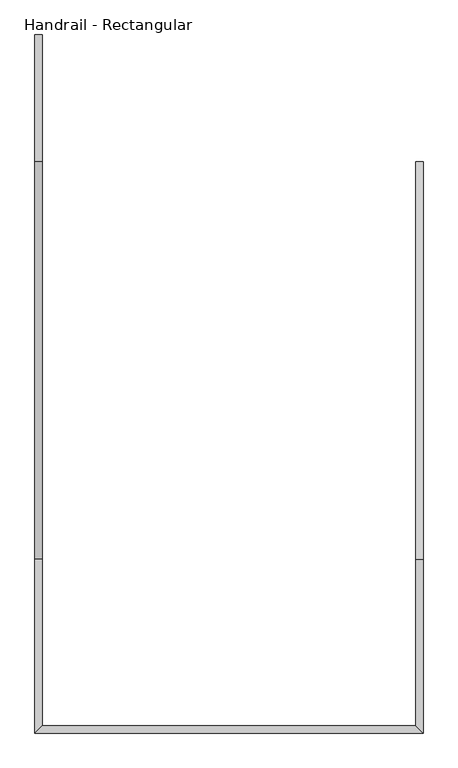
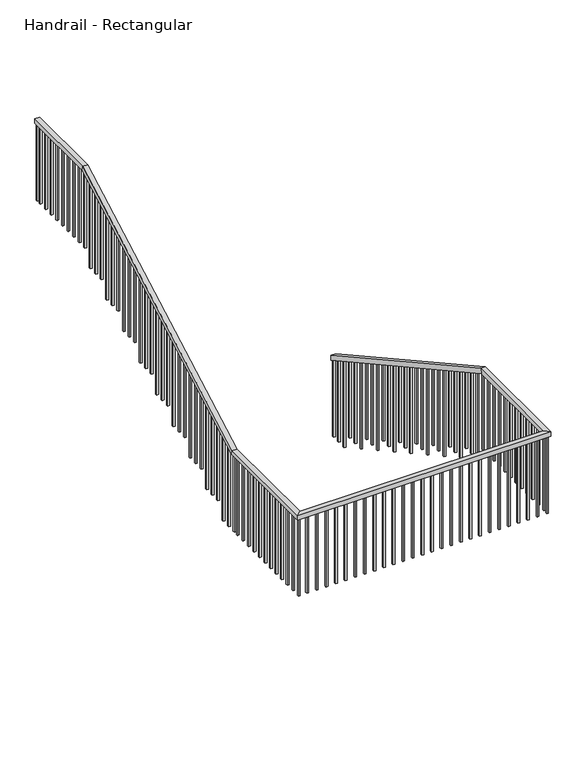
"""IFC4 building model written with IfcOpenShell, lengths in millimetres: railing geometry, Handrail - Rectangular."""

import ifcopenshell
import ifcopenshell.guid

model = None  # the IFC model being written
_history = None  # IfcOwnerHistory: only IFC2X3 demands one
_inside = {}  # id of a spatial element -> (the spatial element, [elements in it])
_under = {}  # id of a project, library or spatial element -> (it, [spatial elements below it])
_declared = {}  # id of a project -> (the project, [libraries it declares])
_typed = {}  # id of a type object -> (the type object, [elements of that type])
_made_of = {}  # id of a material, layer set ... -> (it, [elements and type objects made of it])


def new_model(schema):
    """Start an empty IFC model of exactly this schema.

    Asked for "IFC4X3", IfcOpenShell would pick the latest addendum, in which some entities
    have other attributes; the version numbers below select the first issue.
    IFC2X3 requires an IfcOwnerHistory on every rooted entity: one is made here for all.
    """
    global model, _history
    if schema == "IFC4X3":
        model = ifcopenshell.file(schema_version=(4, 3, 0, 0))
    else:
        model = ifcopenshell.file(schema=schema)
    _inside.clear()
    _under.clear()
    _declared.clear()
    _typed.clear()
    _made_of.clear()
    _history = None
    if model.schema == "IFC2X3":
        org = make("IfcOrganization", Name="unknown")
        user = make(
            "IfcPersonAndOrganization",
            ThePerson=make("IfcPerson", FamilyName="unknown"),
            TheOrganization=org,
        )
        app = make(
            "IfcApplication",
            ApplicationDeveloper=org,
            Version="unknown",
            ApplicationFullName="unknown",
            ApplicationIdentifier="unknown",
        )
        _history = make(
            "IfcOwnerHistory",
            OwningUser=user,
            OwningApplication=app,
            ChangeAction="ADDED",
            CreationDate=0,
        )
    return model


def make(cls, **values):
    """One entity of the class cls with the attributes given. An attribute that is None is left unset."""
    return model.create_entity(
        cls, **{name: value for name, value in values.items() if value is not None}
    )


def rooted(cls, **values):
    """An entity with a GlobalId (a new one), such as an element, a storey or a relation."""
    return make(cls, GlobalId=ifcopenshell.guid.new(), OwnerHistory=_history, **values)


def si_unit(unit_type, name, prefix=None):
    """IfcSIUnit, for example si_unit("LENGTHUNIT", "METRE", prefix="MILLI")."""
    return make("IfcSIUnit", UnitType=unit_type, Prefix=prefix, Name=name)


def assignment(units):
    """IfcUnitAssignment: the units of a project."""
    return None if units is None else make("IfcUnitAssignment", Units=units)


def point(xyz):
    """IfcCartesianPoint."""
    return None if xyz is None else make("IfcCartesianPoint", Coordinates=xyz)


def direction(xyz):
    """IfcDirection."""
    return None if xyz is None else make("IfcDirection", DirectionRatios=xyz)


def frame(location, z_axis=None, x_axis=None):
    """IfcAxis2Placement3D, a coordinate frame: its origin and axes. An axis left out is left unset."""
    return make(
        "IfcAxis2Placement3D",
        Location=point(location),
        Axis=direction(z_axis),
        RefDirection=direction(x_axis),
    )


def origin():
    """The frame at (0, 0, 0) with its axes left unset."""
    return frame((0.0, 0.0, 0.0))


def place(relative_to, where):
    """IfcLocalPlacement: puts the frame where relative to a parent placement (None: the world)."""
    return make(
        "IfcLocalPlacement", PlacementRelTo=relative_to, RelativePlacement=where
    )


def context(
    kind, dimensions, precision=None, world=None, true_north=None, identifier=None
):
    """IfcGeometricRepresentationContext, for example the 3D "Model" context."""
    return make(
        "IfcGeometricRepresentationContext",
        ContextIdentifier=identifier,
        ContextType=kind,
        CoordinateSpaceDimension=dimensions,
        Precision=precision,
        WorldCoordinateSystem=world,
        TrueNorth=true_north,
    )


def project(units=None, contexts=None):
    """IfcProject with its units and contexts."""
    return rooted(
        "IfcProject",
        Name="project",
        RepresentationContexts=contexts,
        UnitsInContext=assignment(units),
    )


def spatial(cls, under=None, at=None, **own):
    """A site, building, storey or space (cls), placed at a placement, below another one or the project."""
    s = rooted(cls, ObjectPlacement=at, **own)
    if under is not None:
        _under.setdefault(under.id(), (under, []))[1].append(s)
    return s


def polyline(points):
    """IfcPolyline through the points."""
    return make("IfcPolyline", Points=[point(p) for p in points])


def outline(outer, holes=None, kind="AREA"):
    """IfcArbitraryClosedProfileDef: a profile drawn as a closed curve; with holes, ...WithVoids."""
    if holes is None:
        return make("IfcArbitraryClosedProfileDef", ProfileType=kind, OuterCurve=outer)
    return make(
        "IfcArbitraryProfileDefWithVoids",
        ProfileType=kind,
        OuterCurve=outer,
        InnerCurves=holes,
    )


def extrude(swept, where, along, depth):
    """IfcExtrudedAreaSolid: the profile swept, set in the frame where, extruded along a direction by depth."""
    return make(
        "IfcExtrudedAreaSolid",
        SweptArea=swept,
        Position=where,
        ExtrudedDirection=direction(along),
        Depth=depth,
    )


def faces_of(points, faces, orient=None, outer=None):
    """IfcFace entities. A face is a list of loops; a loop is a list of indices into points, from 0.

    orient and outer hold one flag for each loop. By default every Orientation is true, the
    first loop of a face is its IfcFaceOuterBound and the others are IfcFaceBound.
    """
    made = []
    for i, loops in enumerate(faces):
        bounds = []
        for j, loop in enumerate(loops):
            is_outer = j == 0 if outer is None else outer[i][j]
            bounds.append(
                make(
                    "IfcFaceOuterBound" if is_outer else "IfcFaceBound",
                    Bound=make("IfcPolyLoop", Polygon=[points[k] for k in loop]),
                    Orientation=True if orient is None else orient[i][j],
                )
            )
        made.append(make("IfcFace", Bounds=bounds))
    return made


def faceted_brep(points, faces, orient=None, outer=None, voids=None):
    """IfcFacetedBrep: a solid bounded by flat faces; with voids (closed shells), ...WithVoids."""
    shared = [point(p) for p in points]
    hull = make("IfcClosedShell", CfsFaces=faces_of(shared, faces, orient, outer))
    if voids is None:
        return make("IfcFacetedBrep", Outer=hull)
    return make(
        "IfcFacetedBrepWithVoids",
        Outer=hull,
        Voids=[
            make(cls, CfsFaces=faces_of(shared, fs, o, b)) for cls, fs, o, b in voids
        ],
    )


def shape(context_of_items, identifier, shape_type, items):
    """IfcShapeRepresentation: the items that make up one representation, for example the "Body"."""
    return make(
        "IfcShapeRepresentation",
        ContextOfItems=context_of_items,
        RepresentationIdentifier=identifier,
        RepresentationType=shape_type,
        Items=items,
    )


def source(mapping_origin, context_of_items, identifier, shape_type, items):
    """IfcRepresentationMap: a shape defined once, which mapped items show again and again."""
    return make(
        "IfcRepresentationMap",
        MappingOrigin=mapping_origin,
        MappedRepresentation=shape(context_of_items, identifier, shape_type, items),
    )


def transform(
    local_origin,
    x_axis=None,
    y_axis=None,
    z_axis=None,
    scale=None,
    scale2=None,
    scale3=None,
    uniform=True,
):
    """IfcCartesianTransformationOperator3D, or its non-uniform kind. x_axis, y_axis, z_axis: its Axis1, 2, 3."""
    if uniform:
        return make(
            "IfcCartesianTransformationOperator3D",
            Axis1=direction(x_axis),
            Axis2=direction(y_axis),
            LocalOrigin=point(local_origin),
            Scale=scale,
            Axis3=direction(z_axis),
        )
    return make(
        "IfcCartesianTransformationOperator3DnonUniform",
        Axis1=direction(x_axis),
        Axis2=direction(y_axis),
        LocalOrigin=point(local_origin),
        Scale=scale,
        Axis3=direction(z_axis),
        Scale2=scale2,
        Scale3=scale3,
    )


def mapped(mapping_source, mapping_target):
    """IfcMappedItem: shows the shape of a source again, moved by a transform."""
    return make(
        "IfcMappedItem", MappingSource=mapping_source, MappingTarget=mapping_target
    )


def made_of(thing, what):
    """Note that an element or type object is made of a material, layer set ...; save() writes the relation."""
    if what is not None:
        _made_of.setdefault(what.id(), (what, []))[1].append(thing)
    return thing


def element(
    cls,
    number,
    at=None,
    inside=None,
    cuts=None,
    type_object=None,
    material=None,
    context=None,
    identifier="Body",
    shape_type=None,
    held_by="IfcProductDefinitionShape",
    body=None,
    shapes=None,
    **own,
):
    """One element of the class cls, such as IfcWall. Its Tag is "e" and its number.

    at: its placement. inside: the storey or other place that contains it. cuts: it is an
    opening in that element (IfcRelVoidsElement). A single representation is given by context,
    identifier, shape_type and body (its items); several are given by shapes. held_by: the class
    of the entity that holds the representations. save() writes the other relations.
    """
    e = rooted(cls, Tag="e%d" % number, ObjectPlacement=at, **own)
    if body is not None:
        shapes = [shape(context, identifier, shape_type, body)]
    if shapes is not None:
        e.Representation = make(held_by, Representations=shapes)
    if inside is not None:
        _inside.setdefault(inside.id(), (inside, []))[1].append(e)
    if cuts is not None:
        rooted(
            "IfcRelVoidsElement", RelatingBuildingElement=cuts, RelatedOpeningElement=e
        )
    if type_object is not None:
        _typed.setdefault(type_object.id(), (type_object, []))[1].append(e)
    return made_of(e, material)


def aggregate(whole, parts):
    """IfcRelAggregates: a whole, such as a stair, and the parts it consists of."""
    return rooted("IfcRelAggregates", RelatingObject=whole, RelatedObjects=parts)


def save(model, path):
    """Write the relations noted so far, then the file.

    IfcRelAggregates (storeys below a building ...), IfcRelContainedInSpatialStructure (elements
    in a storey), IfcRelDefinesByType, IfcRelAssociatesMaterial and IfcRelDeclares: one each for
    every whole, place, type object, material and project.
    """
    for whole, parts in _under.values():
        aggregate(whole, parts)
    for where, things in _inside.values():
        rooted(
            "IfcRelContainedInSpatialStructure",
            RelatedElements=things,
            RelatingStructure=where,
        )
    for kind, things in _typed.values():
        rooted("IfcRelDefinesByType", RelatedObjects=things, RelatingType=kind)
    for what, things in _made_of.values():
        rooted("IfcRelAssociatesMaterial", RelatedObjects=things, RelatingMaterial=what)
    for by, libraries in _declared.values():
        rooted("IfcRelDeclares", RelatingContext=by, RelatedDefinitions=libraries)
    model.write(path)


def handrail_rectangular_0e0fe6d2(model_context):
    return source(origin(), model_context, "Body", "SolidModel", [
        faceted_brep([(-73320.227375, 12915.9, 10449.0921053), (-73269.427375, 12915.9, 10449.0921053), (-73269.427375, 12915.9, 10391.0509841), (-73320.227375, 12915.9, 10391.0509841), (-73320.227375, 10172.7, 11965.0710526), (-73269.427375, 10172.7, 11965.0710526), (-73269.427375, 10159.5970189, 11914.2710526), (-73320.227375, 10159.5970189, 11914.2710526), (-73320.227375, 9023.35, 11965.0710526), (-73269.427375, 8972.55, 11965.0710526), (-73269.427375, 8972.55, 11914.2710526), (-73320.227375, 9023.35, 11914.2710526), (-75898.327375, 9023.35, 11965.0710526), (-75949.127375, 8972.55, 11965.0710526), (-75949.127375, 8972.55, 11914.2710526), (-75898.327375, 9023.35, 11914.2710526), (-75898.327375, 10172.7, 11965.0710526), (-75949.127375, 10172.7, 11965.0710526), (-75949.127375, 10185.8029811, 11914.2710526), (-75898.327375, 10185.8029811, 11914.2710526), (-75898.327375, 12915.9, 13481.05), (-75949.127375, 12915.9, 13481.05), (-75949.127375, 12929.0029811, 13430.25), (-75898.327375, 12929.0029811, 13430.25), (-75898.327375, 13792.2, 13481.05), (-75898.327375, 13792.2, 13430.25), (-75949.127375, 13792.2, 13430.25), (-75949.127375, 13792.2, 13481.05)], [[[0, 1, 2, 3]], [[1, 0, 4, 5]], [[2, 1, 5, 6]], [[3, 2, 6, 7]], [[0, 3, 7, 4]], [[5, 4, 8, 9]], [[6, 5, 9, 10]], [[7, 6, 10, 11]], [[4, 7, 11, 8]], [[9, 8, 12, 13]], [[10, 9, 13, 14]], [[11, 10, 14, 15]], [[8, 11, 15, 12]], [[13, 12, 16, 17]], [[14, 13, 17, 18]], [[15, 14, 18, 19]], [[12, 15, 19, 16]], [[17, 16, 20, 21]], [[18, 17, 21, 22]], [[19, 18, 22, 23]], [[16, 19, 23, 20]], [[24, 25, 26, 27]], [[21, 20, 24, 27]], [[22, 21, 27, 26]], [[23, 22, 26, 25]], [[20, 23, 25, 24]]]),
        extrude(outline(polyline([(-75914.202375, 13719.175), (-75933.252375, 13719.175), (-75933.252375, 13738.225), (-75914.202375, 13738.225), (-75914.202375, 13719.175)])), frame((0.0, 0.0, 12566.65), z_axis=(0.0, 0.0, 1.0), x_axis=(1.0, 0.0, 0.0)), (0.0, 0.0, 1.0), 863.6),
        extrude(outline(polyline([(-75914.202375, 13617.575), (-75933.252375, 13617.575), (-75933.252375, 13636.625), (-75914.202375, 13636.625), (-75914.202375, 13617.575)])), frame((0.0, 0.0, 12566.65), z_axis=(0.0, 0.0, 1.0), x_axis=(1.0, 0.0, 0.0)), (0.0, 0.0, 1.0), 863.6),
        extrude(outline(polyline([(-75914.202375, 13515.975), (-75933.252375, 13515.975), (-75933.252375, 13535.025), (-75914.202375, 13535.025), (-75914.202375, 13515.975)])), frame((0.0, 0.0, 12566.65), z_axis=(0.0, 0.0, 1.0), x_axis=(1.0, 0.0, 0.0)), (0.0, 0.0, 1.0), 863.6),
        extrude(outline(polyline([(-75914.202375, 13414.375), (-75933.252375, 13414.375), (-75933.252375, 13433.425), (-75914.202375, 13433.425), (-75914.202375, 13414.375)])), frame((0.0, 0.0, 12566.65), z_axis=(0.0, 0.0, 1.0), x_axis=(1.0, 0.0, 0.0)), (0.0, 0.0, 1.0), 863.6),
        extrude(outline(polyline([(-75914.202375, 13312.775), (-75933.252375, 13312.775), (-75933.252375, 13331.825), (-75914.202375, 13331.825), (-75914.202375, 13312.775)])), frame((0.0, 0.0, 12566.65), z_axis=(0.0, 0.0, 1.0), x_axis=(1.0, 0.0, 0.0)), (0.0, 0.0, 1.0), 863.6),
        extrude(outline(polyline([(-75914.202375, 13211.175), (-75933.252375, 13211.175), (-75933.252375, 13230.225), (-75914.202375, 13230.225), (-75914.202375, 13211.175)])), frame((0.0, 0.0, 12566.65), z_axis=(0.0, 0.0, 1.0), x_axis=(1.0, 0.0, 0.0)), (0.0, 0.0, 1.0), 863.6),
        extrude(outline(polyline([(-75914.202375, 13109.575), (-75933.252375, 13109.575), (-75933.252375, 13128.625), (-75914.202375, 13128.625), (-75914.202375, 13109.575)])), frame((0.0, 0.0, 12566.65), z_axis=(0.0, 0.0, 1.0), x_axis=(1.0, 0.0, 0.0)), (0.0, 0.0, 1.0), 863.6),
        extrude(outline(polyline([(-75914.202375, 13007.975), (-75933.252375, 13007.975), (-75933.252375, 13027.025), (-75914.202375, 13027.025), (-75914.202375, 13007.975)])), frame((0.0, 0.0, 12566.65), z_axis=(0.0, 0.0, 1.0), x_axis=(1.0, 0.0, 0.0)), (0.0, 0.0, 1.0), 863.6),
        extrude(outline(polyline([(12804.775, 13361.5976946), (12823.825, 13372.1253262), (12823.825, 12398.2078947), (12804.775, 12398.2078947), (12804.775, 13361.5976946)])), frame((-75933.252375, 0.0, 0.0), z_axis=(1.0, 0.0, 0.0), x_axis=(0.0, 1.0, 0.0)), (0.0, 0.0, 1.0), 19.05),
        extrude(outline(polyline([(12703.175, 13305.4503262), (12722.225, 13315.9779578), (12722.225, 12398.2078947), (12703.175, 12398.2078947), (12703.175, 13305.4503262)])), frame((-75933.252375, 0.0, 0.0), z_axis=(1.0, 0.0, 0.0), x_axis=(0.0, 1.0, 0.0)), (0.0, 0.0, 1.0), 19.05),
        extrude(outline(polyline([(12601.575, 13249.3029578), (12620.625, 13259.8305894), (12620.625, 12398.2078947), (12601.575, 12398.2078947), (12601.575, 13249.3029578)])), frame((-75933.252375, 0.0, 0.0), z_axis=(1.0, 0.0, 0.0), x_axis=(0.0, 1.0, 0.0)), (0.0, 0.0, 1.0), 19.05),
        extrude(outline(polyline([(12499.975, 13193.1555894), (12519.025, 13203.6832209), (12519.025, 12229.7657895), (12499.975, 12229.7657895), (12499.975, 13193.1555894)])), frame((-75933.252375, 0.0, 0.0), z_axis=(1.0, 0.0, 0.0), x_axis=(0.0, 1.0, 0.0)), (0.0, 0.0, 1.0), 19.05),
        extrude(outline(polyline([(12398.375, 13137.0082209), (12417.425, 13147.5358525), (12417.425, 12229.7657895), (12398.375, 12229.7657895), (12398.375, 13137.0082209)])), frame((-75933.252375, 0.0, 0.0), z_axis=(1.0, 0.0, 0.0), x_axis=(0.0, 1.0, 0.0)), (0.0, 0.0, 1.0), 19.05),
        extrude(outline(polyline([(12296.775, 13080.8608525), (12315.825, 13091.3884841), (12315.825, 12229.7657895), (12296.775, 12229.7657895), (12296.775, 13080.8608525)])), frame((-75933.252375, 0.0, 0.0), z_axis=(1.0, 0.0, 0.0), x_axis=(0.0, 1.0, 0.0)), (0.0, 0.0, 1.0), 19.05),
        extrude(outline(polyline([(12195.175, 13024.7134841), (12214.225, 13035.2411157), (12214.225, 12061.3236842), (12195.175, 12061.3236842), (12195.175, 13024.7134841)])), frame((-75933.252375, 0.0, 0.0), z_axis=(1.0, 0.0, 0.0), x_axis=(0.0, 1.0, 0.0)), (0.0, 0.0, 1.0), 19.05),
        extrude(outline(polyline([(12093.575, 12968.5661157), (12112.625, 12979.0937473), (12112.625, 12061.3236842), (12093.575, 12061.3236842), (12093.575, 12968.5661157)])), frame((-75933.252375, 0.0, 0.0), z_axis=(1.0, 0.0, 0.0), x_axis=(0.0, 1.0, 0.0)), (0.0, 0.0, 1.0), 19.05),
        extrude(outline(polyline([(11991.975, 12912.4187473), (12011.025, 12922.9463788), (12011.025, 12061.3236842), (11991.975, 12061.3236842), (11991.975, 12912.4187473)])), frame((-75933.252375, 0.0, 0.0), z_axis=(1.0, 0.0, 0.0), x_axis=(0.0, 1.0, 0.0)), (0.0, 0.0, 1.0), 19.05),
        extrude(outline(polyline([(11890.375, 12856.2713788), (11909.425, 12866.7990104), (11909.425, 11892.8815789), (11890.375, 11892.8815789), (11890.375, 12856.2713788)])), frame((-75933.252375, 0.0, 0.0), z_axis=(1.0, 0.0, 0.0), x_axis=(0.0, 1.0, 0.0)), (0.0, 0.0, 1.0), 19.05),
        extrude(outline(polyline([(11788.775, 12800.1240104), (11807.825, 12810.651642), (11807.825, 11892.8815789), (11788.775, 11892.8815789), (11788.775, 12800.1240104)])), frame((-75933.252375, 0.0, 0.0), z_axis=(1.0, 0.0, 0.0), x_axis=(0.0, 1.0, 0.0)), (0.0, 0.0, 1.0), 19.05),
        extrude(outline(polyline([(11687.175, 12743.976642), (11706.225, 12754.5042736), (11706.225, 11892.8815789), (11687.175, 11892.8815789), (11687.175, 12743.976642)])), frame((-75933.252375, 0.0, 0.0), z_axis=(1.0, 0.0, 0.0), x_axis=(0.0, 1.0, 0.0)), (0.0, 0.0, 1.0), 19.05),
        extrude(outline(polyline([(11585.575, 12687.8292736), (11604.625, 12698.3569052), (11604.625, 11724.4394737), (11585.575, 11724.4394737), (11585.575, 12687.8292736)])), frame((-75933.252375, 0.0, 0.0), z_axis=(1.0, 0.0, 0.0), x_axis=(0.0, 1.0, 0.0)), (0.0, 0.0, 1.0), 19.05),
        extrude(outline(polyline([(11483.975, 12631.6819052), (11503.025, 12642.2095367), (11503.025, 11724.4394737), (11483.975, 11724.4394737), (11483.975, 12631.6819052)])), frame((-75933.252375, 0.0, 0.0), z_axis=(1.0, 0.0, 0.0), x_axis=(0.0, 1.0, 0.0)), (0.0, 0.0, 1.0), 19.05),
        extrude(outline(polyline([(11382.375, 12575.5345367), (11401.425, 12586.0621683), (11401.425, 11724.4394737), (11382.375, 11724.4394737), (11382.375, 12575.5345367)])), frame((-75933.252375, 0.0, 0.0), z_axis=(1.0, 0.0, 0.0), x_axis=(0.0, 1.0, 0.0)), (0.0, 0.0, 1.0), 19.05),
        extrude(outline(polyline([(11280.775, 12519.3871683), (11299.825, 12529.9147999), (11299.825, 11555.9973684), (11280.775, 11555.9973684), (11280.775, 12519.3871683)])), frame((-75933.252375, 0.0, 0.0), z_axis=(1.0, 0.0, 0.0), x_axis=(0.0, 1.0, 0.0)), (0.0, 0.0, 1.0), 19.05),
        extrude(outline(polyline([(11179.175, 12463.2397999), (11198.225, 12473.7674315), (11198.225, 11555.9973684), (11179.175, 11555.9973684), (11179.175, 12463.2397999)])), frame((-75933.252375, 0.0, 0.0), z_axis=(1.0, 0.0, 0.0), x_axis=(0.0, 1.0, 0.0)), (0.0, 0.0, 1.0), 19.05),
        extrude(outline(polyline([(11077.575, 12407.0924315), (11096.625, 12417.6200631), (11096.625, 11555.9973684), (11077.575, 11555.9973684), (11077.575, 12407.0924315)])), frame((-75933.252375, 0.0, 0.0), z_axis=(1.0, 0.0, 0.0), x_axis=(0.0, 1.0, 0.0)), (0.0, 0.0, 1.0), 19.05),
        extrude(outline(polyline([(10975.975, 12350.9450631), (10995.025, 12361.4726946), (10995.025, 11387.5552632), (10975.975, 11387.5552632), (10975.975, 12350.9450631)])), frame((-75933.252375, 0.0, 0.0), z_axis=(1.0, 0.0, 0.0), x_axis=(0.0, 1.0, 0.0)), (0.0, 0.0, 1.0), 19.05),
        extrude(outline(polyline([(10874.375, 12294.7976946), (10893.425, 12305.3253262), (10893.425, 11387.5552632), (10874.375, 11387.5552632), (10874.375, 12294.7976946)])), frame((-75933.252375, 0.0, 0.0), z_axis=(1.0, 0.0, 0.0), x_axis=(0.0, 1.0, 0.0)), (0.0, 0.0, 1.0), 19.05),
        extrude(outline(polyline([(10772.775, 12238.6503262), (10791.825, 12249.1779578), (10791.825, 11387.5552632), (10772.775, 11387.5552632), (10772.775, 12238.6503262)])), frame((-75933.252375, 0.0, 0.0), z_axis=(1.0, 0.0, 0.0), x_axis=(0.0, 1.0, 0.0)), (0.0, 0.0, 1.0), 19.05),
        extrude(outline(polyline([(10671.175, 12182.5029578), (10690.225, 12193.0305894), (10690.225, 11219.1131579), (10671.175, 11219.1131579), (10671.175, 12182.5029578)])), frame((-75933.252375, 0.0, 0.0), z_axis=(1.0, 0.0, 0.0), x_axis=(0.0, 1.0, 0.0)), (0.0, 0.0, 1.0), 19.05),
        extrude(outline(polyline([(10569.575, 12126.3555894), (10588.625, 12136.8832209), (10588.625, 11219.1131579), (10569.575, 11219.1131579), (10569.575, 12126.3555894)])), frame((-75933.252375, 0.0, 0.0), z_axis=(1.0, 0.0, 0.0), x_axis=(0.0, 1.0, 0.0)), (0.0, 0.0, 1.0), 19.05),
        extrude(outline(polyline([(10467.975, 12070.2082209), (10487.025, 12080.7358525), (10487.025, 11219.1131579), (10467.975, 11219.1131579), (10467.975, 12070.2082209)])), frame((-75933.252375, 0.0, 0.0), z_axis=(1.0, 0.0, 0.0), x_axis=(0.0, 1.0, 0.0)), (0.0, 0.0, 1.0), 19.05),
        extrude(outline(polyline([(10366.375, 12014.0608525), (10385.425, 12024.5884841), (10385.425, 11050.6710526), (10366.375, 11050.6710526), (10366.375, 12014.0608525)])), frame((-75933.252375, 0.0, 0.0), z_axis=(1.0, 0.0, 0.0), x_axis=(0.0, 1.0, 0.0)), (0.0, 0.0, 1.0), 19.05),
        extrude(outline(polyline([(10264.775, 11957.9134841), (10283.825, 11968.4411157), (10283.825, 11050.6710526), (10264.775, 11050.6710526), (10264.775, 11957.9134841)])), frame((-75933.252375, 0.0, 0.0), z_axis=(1.0, 0.0, 0.0), x_axis=(0.0, 1.0, 0.0)), (0.0, 0.0, 1.0), 19.05),
        extrude(outline(polyline([(-75914.202375, 10106.025), (-75933.252375, 10106.025), (-75933.252375, 10125.075), (-75914.202375, 10125.075), (-75914.202375, 10106.025)])), frame((0.0, 0.0, 11050.6710526), z_axis=(0.0, 0.0, 1.0), x_axis=(1.0, 0.0, 0.0)), (0.0, 0.0, 1.0), 863.6),
        extrude(outline(polyline([(-75914.202375, 10004.425), (-75933.252375, 10004.425), (-75933.252375, 10023.475), (-75914.202375, 10023.475), (-75914.202375, 10004.425)])), frame((0.0, 0.0, 11050.6710526), z_axis=(0.0, 0.0, 1.0), x_axis=(1.0, 0.0, 0.0)), (0.0, 0.0, 1.0), 863.6),
        extrude(outline(polyline([(-75914.202375, 9902.825), (-75933.252375, 9902.825), (-75933.252375, 9921.875), (-75914.202375, 9921.875), (-75914.202375, 9902.825)])), frame((0.0, 0.0, 11050.6710526), z_axis=(0.0, 0.0, 1.0), x_axis=(1.0, 0.0, 0.0)), (0.0, 0.0, 1.0), 863.6),
        extrude(outline(polyline([(-75914.202375, 9801.225), (-75933.252375, 9801.225), (-75933.252375, 9820.275), (-75914.202375, 9820.275), (-75914.202375, 9801.225)])), frame((0.0, 0.0, 11050.6710526), z_axis=(0.0, 0.0, 1.0), x_axis=(1.0, 0.0, 0.0)), (0.0, 0.0, 1.0), 863.6),
        extrude(outline(polyline([(-75914.202375, 9699.625), (-75933.252375, 9699.625), (-75933.252375, 9718.675), (-75914.202375, 9718.675), (-75914.202375, 9699.625)])), frame((0.0, 0.0, 11050.6710526), z_axis=(0.0, 0.0, 1.0), x_axis=(1.0, 0.0, 0.0)), (0.0, 0.0, 1.0), 863.6),
        extrude(outline(polyline([(-75914.202375, 9598.025), (-75933.252375, 9598.025), (-75933.252375, 9617.075), (-75914.202375, 9617.075), (-75914.202375, 9598.025)])), frame((0.0, 0.0, 11050.6710526), z_axis=(0.0, 0.0, 1.0), x_axis=(1.0, 0.0, 0.0)), (0.0, 0.0, 1.0), 863.6),
        extrude(outline(polyline([(-75914.202375, 9496.425), (-75933.252375, 9496.425), (-75933.252375, 9515.475), (-75914.202375, 9515.475), (-75914.202375, 9496.425)])), frame((0.0, 0.0, 11050.6710526), z_axis=(0.0, 0.0, 1.0), x_axis=(1.0, 0.0, 0.0)), (0.0, 0.0, 1.0), 863.6),
        extrude(outline(polyline([(-75914.202375, 9394.825), (-75933.252375, 9394.825), (-75933.252375, 9413.875), (-75914.202375, 9413.875), (-75914.202375, 9394.825)])), frame((0.0, 0.0, 11050.6710526), z_axis=(0.0, 0.0, 1.0), x_axis=(1.0, 0.0, 0.0)), (0.0, 0.0, 1.0), 863.6),
        extrude(outline(polyline([(-75914.202375, 9293.225), (-75933.252375, 9293.225), (-75933.252375, 9312.275), (-75914.202375, 9312.275), (-75914.202375, 9293.225)])), frame((0.0, 0.0, 11050.6710526), z_axis=(0.0, 0.0, 1.0), x_axis=(1.0, 0.0, 0.0)), (0.0, 0.0, 1.0), 863.6),
        extrude(outline(polyline([(-75914.202375, 9191.625), (-75933.252375, 9191.625), (-75933.252375, 9210.675), (-75914.202375, 9210.675), (-75914.202375, 9191.625)])), frame((0.0, 0.0, 11050.6710526), z_axis=(0.0, 0.0, 1.0), x_axis=(1.0, 0.0, 0.0)), (0.0, 0.0, 1.0), 863.6),
        extrude(outline(polyline([(-75914.202375, 9090.025), (-75933.252375, 9090.025), (-75933.252375, 9109.075), (-75914.202375, 9109.075), (-75914.202375, 9090.025)])), frame((0.0, 0.0, 11050.6710526), z_axis=(0.0, 0.0, 1.0), x_axis=(1.0, 0.0, 0.0)), (0.0, 0.0, 1.0), 863.6),
        extrude(outline(polyline([(-75825.302375, 9007.475), (-75825.302375, 8988.425), (-75844.352375, 8988.425), (-75844.352375, 9007.475), (-75825.302375, 9007.475)])), frame((0.0, 0.0, 11050.6710526), z_axis=(0.0, 0.0, 1.0), x_axis=(1.0, 0.0, 0.0)), (0.0, 0.0, 1.0), 863.6),
        extrude(outline(polyline([(-75723.702375, 9007.475), (-75723.702375, 8988.425), (-75742.752375, 8988.425), (-75742.752375, 9007.475), (-75723.702375, 9007.475)])), frame((0.0, 0.0, 11050.6710526), z_axis=(0.0, 0.0, 1.0), x_axis=(1.0, 0.0, 0.0)), (0.0, 0.0, 1.0), 863.6),
        extrude(outline(polyline([(-75622.102375, 9007.475), (-75622.102375, 8988.425), (-75641.152375, 8988.425), (-75641.152375, 9007.475), (-75622.102375, 9007.475)])), frame((0.0, 0.0, 11050.6710526), z_axis=(0.0, 0.0, 1.0), x_axis=(1.0, 0.0, 0.0)), (0.0, 0.0, 1.0), 863.6),
        extrude(outline(polyline([(-75520.502375, 9007.475), (-75520.502375, 8988.425), (-75539.552375, 8988.425), (-75539.552375, 9007.475), (-75520.502375, 9007.475)])), frame((0.0, 0.0, 11050.6710526), z_axis=(0.0, 0.0, 1.0), x_axis=(1.0, 0.0, 0.0)), (0.0, 0.0, 1.0), 863.6),
        extrude(outline(polyline([(-75418.902375, 9007.475), (-75418.902375, 8988.425), (-75437.952375, 8988.425), (-75437.952375, 9007.475), (-75418.902375, 9007.475)])), frame((0.0, 0.0, 11050.6710526), z_axis=(0.0, 0.0, 1.0), x_axis=(1.0, 0.0, 0.0)), (0.0, 0.0, 1.0), 863.6),
        extrude(outline(polyline([(-75317.302375, 9007.475), (-75317.302375, 8988.425), (-75336.352375, 8988.425), (-75336.352375, 9007.475), (-75317.302375, 9007.475)])), frame((0.0, 0.0, 11050.6710526), z_axis=(0.0, 0.0, 1.0), x_axis=(1.0, 0.0, 0.0)), (0.0, 0.0, 1.0), 863.6),
        extrude(outline(polyline([(-75215.702375, 9007.475), (-75215.702375, 8988.425), (-75234.752375, 8988.425), (-75234.752375, 9007.475), (-75215.702375, 9007.475)])), frame((0.0, 0.0, 11050.6710526), z_axis=(0.0, 0.0, 1.0), x_axis=(1.0, 0.0, 0.0)), (0.0, 0.0, 1.0), 863.6),
        extrude(outline(polyline([(-75114.102375, 9007.475), (-75114.102375, 8988.425), (-75133.152375, 8988.425), (-75133.152375, 9007.475), (-75114.102375, 9007.475)])), frame((0.0, 0.0, 11050.6710526), z_axis=(0.0, 0.0, 1.0), x_axis=(1.0, 0.0, 0.0)), (0.0, 0.0, 1.0), 863.6),
        extrude(outline(polyline([(-75012.502375, 9007.475), (-75012.502375, 8988.425), (-75031.552375, 8988.425), (-75031.552375, 9007.475), (-75012.502375, 9007.475)])), frame((0.0, 0.0, 11050.6710526), z_axis=(0.0, 0.0, 1.0), x_axis=(1.0, 0.0, 0.0)), (0.0, 0.0, 1.0), 863.6),
        extrude(outline(polyline([(-74910.902375, 9007.475), (-74910.902375, 8988.425), (-74929.952375, 8988.425), (-74929.952375, 9007.475), (-74910.902375, 9007.475)])), frame((0.0, 0.0, 11050.6710526), z_axis=(0.0, 0.0, 1.0), x_axis=(1.0, 0.0, 0.0)), (0.0, 0.0, 1.0), 863.6),
        extrude(outline(polyline([(-74809.302375, 9007.475), (-74809.302375, 8988.425), (-74828.352375, 8988.425), (-74828.352375, 9007.475), (-74809.302375, 9007.475)])), frame((0.0, 0.0, 11050.6710526), z_axis=(0.0, 0.0, 1.0), x_axis=(1.0, 0.0, 0.0)), (0.0, 0.0, 1.0), 863.6),
        extrude(outline(polyline([(-74707.702375, 9007.475), (-74707.702375, 8988.425), (-74726.752375, 8988.425), (-74726.752375, 9007.475), (-74707.702375, 9007.475)])), frame((0.0, 0.0, 11050.6710526), z_axis=(0.0, 0.0, 1.0), x_axis=(1.0, 0.0, 0.0)), (0.0, 0.0, 1.0), 863.6),
        extrude(outline(polyline([(-74606.102375, 9007.475), (-74606.102375, 8988.425), (-74625.152375, 8988.425), (-74625.152375, 9007.475), (-74606.102375, 9007.475)])), frame((0.0, 0.0, 11050.6710526), z_axis=(0.0, 0.0, 1.0), x_axis=(1.0, 0.0, 0.0)), (0.0, 0.0, 1.0), 863.6),
        extrude(outline(polyline([(-74504.502375, 9007.475), (-74504.502375, 8988.425), (-74523.552375, 8988.425), (-74523.552375, 9007.475), (-74504.502375, 9007.475)])), frame((0.0, 0.0, 11050.6710526), z_axis=(0.0, 0.0, 1.0), x_axis=(1.0, 0.0, 0.0)), (0.0, 0.0, 1.0), 863.6),
        extrude(outline(polyline([(-74402.902375, 9007.475), (-74402.902375, 8988.425), (-74421.952375, 8988.425), (-74421.952375, 9007.475), (-74402.902375, 9007.475)])), frame((0.0, 0.0, 11050.6710526), z_axis=(0.0, 0.0, 1.0), x_axis=(1.0, 0.0, 0.0)), (0.0, 0.0, 1.0), 863.6),
        extrude(outline(polyline([(-74301.302375, 9007.475), (-74301.302375, 8988.425), (-74320.352375, 8988.425), (-74320.352375, 9007.475), (-74301.302375, 9007.475)])), frame((0.0, 0.0, 11050.6710526), z_axis=(0.0, 0.0, 1.0), x_axis=(1.0, 0.0, 0.0)), (0.0, 0.0, 1.0), 863.6),
        extrude(outline(polyline([(-74199.702375, 9007.475), (-74199.702375, 8988.425), (-74218.752375, 8988.425), (-74218.752375, 9007.475), (-74199.702375, 9007.475)])), frame((0.0, 0.0, 11050.6710526), z_axis=(0.0, 0.0, 1.0), x_axis=(1.0, 0.0, 0.0)), (0.0, 0.0, 1.0), 863.6),
        extrude(outline(polyline([(-74098.102375, 9007.475), (-74098.102375, 8988.425), (-74117.152375, 8988.425), (-74117.152375, 9007.475), (-74098.102375, 9007.475)])), frame((0.0, 0.0, 11050.6710526), z_axis=(0.0, 0.0, 1.0), x_axis=(1.0, 0.0, 0.0)), (0.0, 0.0, 1.0), 863.6),
        extrude(outline(polyline([(-73996.502375, 9007.475), (-73996.502375, 8988.425), (-74015.552375, 8988.425), (-74015.552375, 9007.475), (-73996.502375, 9007.475)])), frame((0.0, 0.0, 11050.6710526), z_axis=(0.0, 0.0, 1.0), x_axis=(1.0, 0.0, 0.0)), (0.0, 0.0, 1.0), 863.6),
        extrude(outline(polyline([(-73894.902375, 9007.475), (-73894.902375, 8988.425), (-73913.952375, 8988.425), (-73913.952375, 9007.475), (-73894.902375, 9007.475)])), frame((0.0, 0.0, 11050.6710526), z_axis=(0.0, 0.0, 1.0), x_axis=(1.0, 0.0, 0.0)), (0.0, 0.0, 1.0), 863.6),
        extrude(outline(polyline([(-73793.302375, 9007.475), (-73793.302375, 8988.425), (-73812.352375, 8988.425), (-73812.352375, 9007.475), (-73793.302375, 9007.475)])), frame((0.0, 0.0, 11050.6710526), z_axis=(0.0, 0.0, 1.0), x_axis=(1.0, 0.0, 0.0)), (0.0, 0.0, 1.0), 863.6),
        extrude(outline(polyline([(-73691.702375, 9007.475), (-73691.702375, 8988.425), (-73710.752375, 8988.425), (-73710.752375, 9007.475), (-73691.702375, 9007.475)])), frame((0.0, 0.0, 11050.6710526), z_axis=(0.0, 0.0, 1.0), x_axis=(1.0, 0.0, 0.0)), (0.0, 0.0, 1.0), 863.6),
        extrude(outline(polyline([(-73590.102375, 9007.475), (-73590.102375, 8988.425), (-73609.152375, 8988.425), (-73609.152375, 9007.475), (-73590.102375, 9007.475)])), frame((0.0, 0.0, 11050.6710526), z_axis=(0.0, 0.0, 1.0), x_axis=(1.0, 0.0, 0.0)), (0.0, 0.0, 1.0), 863.6),
        extrude(outline(polyline([(-73488.502375, 9007.475), (-73488.502375, 8988.425), (-73507.552375, 8988.425), (-73507.552375, 9007.475), (-73488.502375, 9007.475)])), frame((0.0, 0.0, 11050.6710526), z_axis=(0.0, 0.0, 1.0), x_axis=(1.0, 0.0, 0.0)), (0.0, 0.0, 1.0), 863.6),
        extrude(outline(polyline([(-73386.902375, 9007.475), (-73386.902375, 8988.425), (-73405.952375, 8988.425), (-73405.952375, 9007.475), (-73386.902375, 9007.475)])), frame((0.0, 0.0, 11050.6710526), z_axis=(0.0, 0.0, 1.0), x_axis=(1.0, 0.0, 0.0)), (0.0, 0.0, 1.0), 863.6),
        extrude(outline(polyline([(-73304.352375, 9064.625), (-73285.302375, 9064.625), (-73285.302375, 9045.575), (-73304.352375, 9045.575), (-73304.352375, 9064.625)])), frame((0.0, 0.0, 11050.6710526), z_axis=(0.0, 0.0, 1.0), x_axis=(1.0, 0.0, 0.0)), (0.0, 0.0, 1.0), 863.6),
        extrude(outline(polyline([(-73304.352375, 9166.225), (-73285.302375, 9166.225), (-73285.302375, 9147.175), (-73304.352375, 9147.175), (-73304.352375, 9166.225)])), frame((0.0, 0.0, 11050.6710526), z_axis=(0.0, 0.0, 1.0), x_axis=(1.0, 0.0, 0.0)), (0.0, 0.0, 1.0), 863.6),
        extrude(outline(polyline([(-73304.352375, 9267.825), (-73285.302375, 9267.825), (-73285.302375, 9248.775), (-73304.352375, 9248.775), (-73304.352375, 9267.825)])), frame((0.0, 0.0, 11050.6710526), z_axis=(0.0, 0.0, 1.0), x_axis=(1.0, 0.0, 0.0)), (0.0, 0.0, 1.0), 863.6),
        extrude(outline(polyline([(-73304.352375, 9369.425), (-73285.302375, 9369.425), (-73285.302375, 9350.375), (-73304.352375, 9350.375), (-73304.352375, 9369.425)])), frame((0.0, 0.0, 11050.6710526), z_axis=(0.0, 0.0, 1.0), x_axis=(1.0, 0.0, 0.0)), (0.0, 0.0, 1.0), 863.6),
        extrude(outline(polyline([(-73304.352375, 9471.025), (-73285.302375, 9471.025), (-73285.302375, 9451.975), (-73304.352375, 9451.975), (-73304.352375, 9471.025)])), frame((0.0, 0.0, 11050.6710526), z_axis=(0.0, 0.0, 1.0), x_axis=(1.0, 0.0, 0.0)), (0.0, 0.0, 1.0), 863.6),
        extrude(outline(polyline([(-73304.352375, 9572.625), (-73285.302375, 9572.625), (-73285.302375, 9553.575), (-73304.352375, 9553.575), (-73304.352375, 9572.625)])), frame((0.0, 0.0, 11050.6710526), z_axis=(0.0, 0.0, 1.0), x_axis=(1.0, 0.0, 0.0)), (0.0, 0.0, 1.0), 863.6),
        extrude(outline(polyline([(-73304.352375, 9674.225), (-73285.302375, 9674.225), (-73285.302375, 9655.175), (-73304.352375, 9655.175), (-73304.352375, 9674.225)])), frame((0.0, 0.0, 11050.6710526), z_axis=(0.0, 0.0, 1.0), x_axis=(1.0, 0.0, 0.0)), (0.0, 0.0, 1.0), 863.6),
        extrude(outline(polyline([(-73304.352375, 9775.825), (-73285.302375, 9775.825), (-73285.302375, 9756.775), (-73304.352375, 9756.775), (-73304.352375, 9775.825)])), frame((0.0, 0.0, 11050.6710526), z_axis=(0.0, 0.0, 1.0), x_axis=(1.0, 0.0, 0.0)), (0.0, 0.0, 1.0), 863.6),
        extrude(outline(polyline([(-73304.352375, 9877.425), (-73285.302375, 9877.425), (-73285.302375, 9858.375), (-73304.352375, 9858.375), (-73304.352375, 9877.425)])), frame((0.0, 0.0, 11050.6710526), z_axis=(0.0, 0.0, 1.0), x_axis=(1.0, 0.0, 0.0)), (0.0, 0.0, 1.0), 863.6),
        extrude(outline(polyline([(-73304.352375, 9979.025), (-73285.302375, 9979.025), (-73285.302375, 9959.975), (-73304.352375, 9959.975), (-73304.352375, 9979.025)])), frame((0.0, 0.0, 11050.6710526), z_axis=(0.0, 0.0, 1.0), x_axis=(1.0, 0.0, 0.0)), (0.0, 0.0, 1.0), 863.6),
        extrude(outline(polyline([(-73304.352375, 10080.625), (-73285.302375, 10080.625), (-73285.302375, 10061.575), (-73304.352375, 10061.575), (-73304.352375, 10080.625)])), frame((0.0, 0.0, 11050.6710526), z_axis=(0.0, 0.0, 1.0), x_axis=(1.0, 0.0, 0.0)), (0.0, 0.0, 1.0), 863.6),
        extrude(outline(polyline([(10264.775, 11856.1463788), (10283.825, 11845.6187473), (10283.825, 10882.2289474), (10264.775, 10882.2289474), (10264.775, 11856.1463788)])), frame((-73304.352375, 0.0, 0.0), z_axis=(1.0, 0.0, 0.0), x_axis=(0.0, 1.0, 0.0)), (0.0, 0.0, 1.0), 19.05),
        extrude(outline(polyline([(10366.375, 11799.9990104), (10385.425, 11789.4713788), (10385.425, 10882.2289474), (10366.375, 10882.2289474), (10366.375, 11799.9990104)])), frame((-73304.352375, 0.0, 0.0), z_axis=(1.0, 0.0, 0.0), x_axis=(0.0, 1.0, 0.0)), (0.0, 0.0, 1.0), 19.05),
        extrude(outline(polyline([(10467.975, 11743.851642), (10487.025, 11733.3240104), (10487.025, 10882.2289474), (10467.975, 10882.2289474), (10467.975, 11743.851642)])), frame((-73304.352375, 0.0, 0.0), z_axis=(1.0, 0.0, 0.0), x_axis=(0.0, 1.0, 0.0)), (0.0, 0.0, 1.0), 19.05),
        extrude(outline(polyline([(10569.575, 11687.7042736), (10588.625, 11677.176642), (10588.625, 10713.7868421), (10569.575, 10713.7868421), (10569.575, 11687.7042736)])), frame((-73304.352375, 0.0, 0.0), z_axis=(1.0, 0.0, 0.0), x_axis=(0.0, 1.0, 0.0)), (0.0, 0.0, 1.0), 19.05),
        extrude(outline(polyline([(10671.175, 11631.5569052), (10690.225, 11621.0292736), (10690.225, 10713.7868421), (10671.175, 10713.7868421), (10671.175, 11631.5569052)])), frame((-73304.352375, 0.0, 0.0), z_axis=(1.0, 0.0, 0.0), x_axis=(0.0, 1.0, 0.0)), (0.0, 0.0, 1.0), 19.05),
        extrude(outline(polyline([(10772.775, 11575.4095367), (10791.825, 11564.8819052), (10791.825, 10713.7868421), (10772.775, 10713.7868421), (10772.775, 11575.4095367)])), frame((-73304.352375, 0.0, 0.0), z_axis=(1.0, 0.0, 0.0), x_axis=(0.0, 1.0, 0.0)), (0.0, 0.0, 1.0), 19.05),
        extrude(outline(polyline([(10874.375, 11519.2621683), (10893.425, 11508.7345367), (10893.425, 10545.3447368), (10874.375, 10545.3447368), (10874.375, 11519.2621683)])), frame((-73304.352375, 0.0, 0.0), z_axis=(1.0, 0.0, 0.0), x_axis=(0.0, 1.0, 0.0)), (0.0, 0.0, 1.0), 19.05),
        extrude(outline(polyline([(10975.975, 11463.1147999), (10995.025, 11452.5871683), (10995.025, 10545.3447368), (10975.975, 10545.3447368), (10975.975, 11463.1147999)])), frame((-73304.352375, 0.0, 0.0), z_axis=(1.0, 0.0, 0.0), x_axis=(0.0, 1.0, 0.0)), (0.0, 0.0, 1.0), 19.05),
        extrude(outline(polyline([(11077.575, 11406.9674315), (11096.625, 11396.4397999), (11096.625, 10545.3447368), (11077.575, 10545.3447368), (11077.575, 11406.9674315)])), frame((-73304.352375, 0.0, 0.0), z_axis=(1.0, 0.0, 0.0), x_axis=(0.0, 1.0, 0.0)), (0.0, 0.0, 1.0), 19.05),
        extrude(outline(polyline([(11179.175, 11350.8200631), (11198.225, 11340.2924315), (11198.225, 10376.9026316), (11179.175, 10376.9026316), (11179.175, 11350.8200631)])), frame((-73304.352375, 0.0, 0.0), z_axis=(1.0, 0.0, 0.0), x_axis=(0.0, 1.0, 0.0)), (0.0, 0.0, 1.0), 19.05),
        extrude(outline(polyline([(11280.775, 11294.6726946), (11299.825, 11284.1450631), (11299.825, 10376.9026316), (11280.775, 10376.9026316), (11280.775, 11294.6726946)])), frame((-73304.352375, 0.0, 0.0), z_axis=(1.0, 0.0, 0.0), x_axis=(0.0, 1.0, 0.0)), (0.0, 0.0, 1.0), 19.05),
        extrude(outline(polyline([(11382.375, 11238.5253262), (11401.425, 11227.9976946), (11401.425, 10376.9026316), (11382.375, 10376.9026316), (11382.375, 11238.5253262)])), frame((-73304.352375, 0.0, 0.0), z_axis=(1.0, 0.0, 0.0), x_axis=(0.0, 1.0, 0.0)), (0.0, 0.0, 1.0), 19.05),
        extrude(outline(polyline([(11483.975, 11182.3779578), (11503.025, 11171.8503262), (11503.025, 10208.4605263), (11483.975, 10208.4605263), (11483.975, 11182.3779578)])), frame((-73304.352375, 0.0, 0.0), z_axis=(1.0, 0.0, 0.0), x_axis=(0.0, 1.0, 0.0)), (0.0, 0.0, 1.0), 19.05),
        extrude(outline(polyline([(11585.575, 11126.2305894), (11604.625, 11115.7029578), (11604.625, 10208.4605263), (11585.575, 10208.4605263), (11585.575, 11126.2305894)])), frame((-73304.352375, 0.0, 0.0), z_axis=(1.0, 0.0, 0.0), x_axis=(0.0, 1.0, 0.0)), (0.0, 0.0, 1.0), 19.05),
        extrude(outline(polyline([(11687.175, 11070.0832209), (11706.225, 11059.5555894), (11706.225, 10208.4605263), (11687.175, 10208.4605263), (11687.175, 11070.0832209)])), frame((-73304.352375, 0.0, 0.0), z_axis=(1.0, 0.0, 0.0), x_axis=(0.0, 1.0, 0.0)), (0.0, 0.0, 1.0), 19.05),
        extrude(outline(polyline([(11788.775, 11013.9358525), (11807.825, 11003.4082209), (11807.825, 10040.0184211), (11788.775, 10040.0184211), (11788.775, 11013.9358525)])), frame((-73304.352375, 0.0, 0.0), z_axis=(1.0, 0.0, 0.0), x_axis=(0.0, 1.0, 0.0)), (0.0, 0.0, 1.0), 19.05),
        extrude(outline(polyline([(11890.375, 10957.7884841), (11909.425, 10947.2608525), (11909.425, 10040.0184211), (11890.375, 10040.0184211), (11890.375, 10957.7884841)])), frame((-73304.352375, 0.0, 0.0), z_axis=(1.0, 0.0, 0.0), x_axis=(0.0, 1.0, 0.0)), (0.0, 0.0, 1.0), 19.05),
        extrude(outline(polyline([(11991.975, 10901.6411157), (12011.025, 10891.1134841), (12011.025, 10040.0184211), (11991.975, 10040.0184211), (11991.975, 10901.6411157)])), frame((-73304.352375, 0.0, 0.0), z_axis=(1.0, 0.0, 0.0), x_axis=(0.0, 1.0, 0.0)), (0.0, 0.0, 1.0), 19.05),
        extrude(outline(polyline([(12093.575, 10845.4937473), (12112.625, 10834.9661157), (12112.625, 9871.5763158), (12093.575, 9871.5763158), (12093.575, 10845.4937473)])), frame((-73304.352375, 0.0, 0.0), z_axis=(1.0, 0.0, 0.0), x_axis=(0.0, 1.0, 0.0)), (0.0, 0.0, 1.0), 19.05),
        extrude(outline(polyline([(12195.175, 10789.3463788), (12214.225, 10778.8187473), (12214.225, 9871.5763158), (12195.175, 9871.5763158), (12195.175, 10789.3463788)])), frame((-73304.352375, 0.0, 0.0), z_axis=(1.0, 0.0, 0.0), x_axis=(0.0, 1.0, 0.0)), (0.0, 0.0, 1.0), 19.05),
        extrude(outline(polyline([(12296.775, 10733.1990104), (12315.825, 10722.6713788), (12315.825, 9871.5763158), (12296.775, 9871.5763158), (12296.775, 10733.1990104)])), frame((-73304.352375, 0.0, 0.0), z_axis=(1.0, 0.0, 0.0), x_axis=(0.0, 1.0, 0.0)), (0.0, 0.0, 1.0), 19.05),
        extrude(outline(polyline([(12398.375, 10677.051642), (12417.425, 10666.5240104), (12417.425, 9703.1342105), (12398.375, 9703.1342105), (12398.375, 10677.051642)])), frame((-73304.352375, 0.0, 0.0), z_axis=(1.0, 0.0, 0.0), x_axis=(0.0, 1.0, 0.0)), (0.0, 0.0, 1.0), 19.05),
        extrude(outline(polyline([(12499.975, 10620.9042736), (12519.025, 10610.376642), (12519.025, 9703.1342105), (12499.975, 9703.1342105), (12499.975, 10620.9042736)])), frame((-73304.352375, 0.0, 0.0), z_axis=(1.0, 0.0, 0.0), x_axis=(0.0, 1.0, 0.0)), (0.0, 0.0, 1.0), 19.05),
        extrude(outline(polyline([(12601.575, 10564.7569052), (12620.625, 10554.2292736), (12620.625, 9703.1342105), (12601.575, 9703.1342105), (12601.575, 10564.7569052)])), frame((-73304.352375, 0.0, 0.0), z_axis=(1.0, 0.0, 0.0), x_axis=(0.0, 1.0, 0.0)), (0.0, 0.0, 1.0), 19.05),
        extrude(outline(polyline([(12703.175, 10508.6095367), (12722.225, 10498.0819052), (12722.225, 9534.6921053), (12703.175, 9534.6921053), (12703.175, 10508.6095367)])), frame((-73304.352375, 0.0, 0.0), z_axis=(1.0, 0.0, 0.0), x_axis=(0.0, 1.0, 0.0)), (0.0, 0.0, 1.0), 19.05),
        extrude(outline(polyline([(12804.775, 10452.4621683), (12823.825, 10441.9345367), (12823.825, 9534.6921053), (12804.775, 9534.6921053), (12804.775, 10452.4621683)])), frame((-73304.352375, 0.0, 0.0), z_axis=(1.0, 0.0, 0.0), x_axis=(0.0, 1.0, 0.0)), (0.0, 0.0, 1.0), 19.05),
        extrude(outline(polyline([(12906.375, 13417.7450631), (12925.425, 13428.2726946), (12925.425, 12566.65), (12906.375, 12566.65), (12906.375, 13417.7450631)])), frame((-75933.252375, 0.0, 0.0), z_axis=(1.0, 0.0, 0.0), x_axis=(0.0, 1.0, 0.0)), (0.0, 0.0, 1.0), 19.05),
        extrude(outline(polyline([(-75914.202375, 10163.175), (-75933.252375, 10163.175), (-75933.252375, 10182.225), (-75914.202375, 10182.225), (-75914.202375, 10163.175)])), frame((0.0, 0.0, 11050.6710526), z_axis=(0.0, 0.0, 1.0), x_axis=(1.0, 0.0, 0.0)), (0.0, 0.0, 1.0), 863.6),
        extrude(outline(polyline([(-75914.202375, 9007.475), (-75914.202375, 8988.425), (-75933.252375, 8988.425), (-75933.252375, 9007.475), (-75914.202375, 9007.475)])), frame((0.0, 0.0, 11050.6710526), z_axis=(0.0, 0.0, 1.0), x_axis=(1.0, 0.0, 0.0)), (0.0, 0.0, 1.0), 863.6),
        extrude(outline(polyline([(-73304.352375, 9007.475), (-73285.302375, 9007.475), (-73285.302375, 8988.425), (-73304.352375, 8988.425), (-73304.352375, 9007.475)])), frame((0.0, 0.0, 11050.6710526), z_axis=(0.0, 0.0, 1.0), x_axis=(1.0, 0.0, 0.0)), (0.0, 0.0, 1.0), 863.6),
        extrude(outline(polyline([(10163.175, 11912.2937473), (10182.225, 11901.7661157), (10182.225, 11050.6710526), (10163.175, 11050.6710526), (10163.175, 11912.2937473)])), frame((-73304.352375, 0.0, 0.0), z_axis=(1.0, 0.0, 0.0), x_axis=(0.0, 1.0, 0.0)), (0.0, 0.0, 1.0), 19.05),
        extrude(outline(polyline([(-75914.202375, 13773.15), (-75933.252375, 13773.15), (-75933.252375, 13792.2), (-75914.202375, 13792.2), (-75914.202375, 13773.15)])), frame((0.0, 0.0, 12566.65), z_axis=(0.0, 0.0, 1.0), x_axis=(1.0, 0.0, 0.0)), (0.0, 0.0, 1.0), 863.6),
        extrude(outline(polyline([(12896.85, 10401.5786157), (12915.9, 10391.0509841), (12915.9, 9534.6921053), (12896.85, 9534.6921053), (12896.85, 10401.5786157)])), frame((-73304.352375, 0.0, 0.0), z_axis=(1.0, 0.0, 0.0), x_axis=(0.0, 1.0, 0.0)), (0.0, 0.0, 1.0), 19.05),
    ])


if __name__ == "__main__":
    model = new_model("IFC4")
    model_context = context("Model", 3, world=origin())
    ifc_project = project(units=[si_unit("LENGTHUNIT", "METRE", prefix="MILLI")], contexts=[model_context])
    site = spatial("IfcSite", under=ifc_project)
    building = spatial("IfcBuilding", under=site)
    placement = place(None, origin())
    handrail_rectangular_shape = handrail_rectangular_0e0fe6d2(model_context)
    element("IfcRailing", 1, ObjectType="Handrail - Rectangular", at=placement, inside=building, context=model_context, shape_type="MappedRepresentation", body=[
        mapped(handrail_rectangular_shape, transform((0.0, 0.0, 0.0), x_axis=(1.0, 0.0, 0.0), y_axis=(0.0, 1.0, 0.0), z_axis=(0.0, 0.0, 1.0))),
    ])
    save(model, "model.ifc")
